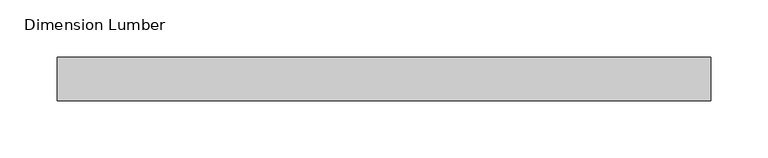
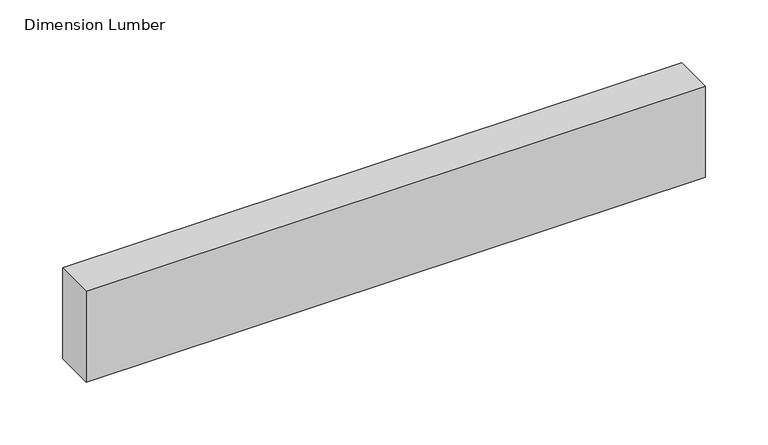
"""IFC4 building model written with IfcOpenShell, lengths in millimetres: beam geometry, Dimension Lumber : Roof Lumbers."""

from ifc_helpers import new_model, si_unit, frame, origin, place, context, project, spatial, polyline, outline, extrude, source, transform, mapped, element, save


def dimension_lumber_d546034e(model_context):
    return source(origin(), model_context, "Body", "SweptSolid", [
        extrude(outline(polyline([(295.275, 19.05), (295.275, -19.05), (-276.225, -19.05), (-276.225, 19.05), (295.275, 19.05)])), frame((0.0, 0.0, -44.45), z_axis=(0.0, 0.0, 1.0), x_axis=(1.0, 0.0, 0.0)), (0.0, 0.0, 1.0), 88.9),
    ])


if __name__ == "__main__":
    model = new_model("IFC4")
    model_context = context("Model", 3, world=origin())
    ifc_project = project(units=[si_unit("LENGTHUNIT", "METRE", prefix="MILLI")], contexts=[model_context])
    site = spatial("IfcSite", under=ifc_project)
    building = spatial("IfcBuilding", under=site)
    placement = place(None, origin())
    dimension_lumber_shape = dimension_lumber_d546034e(model_context)
    element("IfcBeam", 1, ObjectType="Dimension Lumber : Roof Lumbers", at=placement, inside=building, context=model_context, shape_type="MappedRepresentation", body=[
        mapped(dimension_lumber_shape, transform((0.0, 0.0, 0.0), x_axis=(1.0, 0.0, 0.0), y_axis=(0.0, 1.0, 0.0), z_axis=(0.0, 0.0, 1.0))),
    ])
    save(model, "model.ifc")

# Revit data of these elements
# Type "Dimension Lumber : Roof Lumbers"
#   Assembly Code = "B10"
#   A = 0.0364583 SF
#   Length [instance default] = 5' - 0"
#   b = 0' - 1 1/2"
#   d = 0' - 3 1/2"
#   Structural Material [instance default] = Softwood, Lumber
# Element 1 (IfcBeam, "Dimension Lumber : Roof Lumbers")
#   Structural Material = Douglas Fir #2
#   Materials on its faces: "Douglas Fir #2"
# Materials
#   "Softwood, Lumber": class "Wood", colour RGB 223 192 134, transparency 0, Description = "Pinus Echinata", Cost = 0
#   "Douglas Fir #2": class "Wood", colour RGB 223 192 134, transparency 0, Description = "Pinus Echinata", Cost = 0
